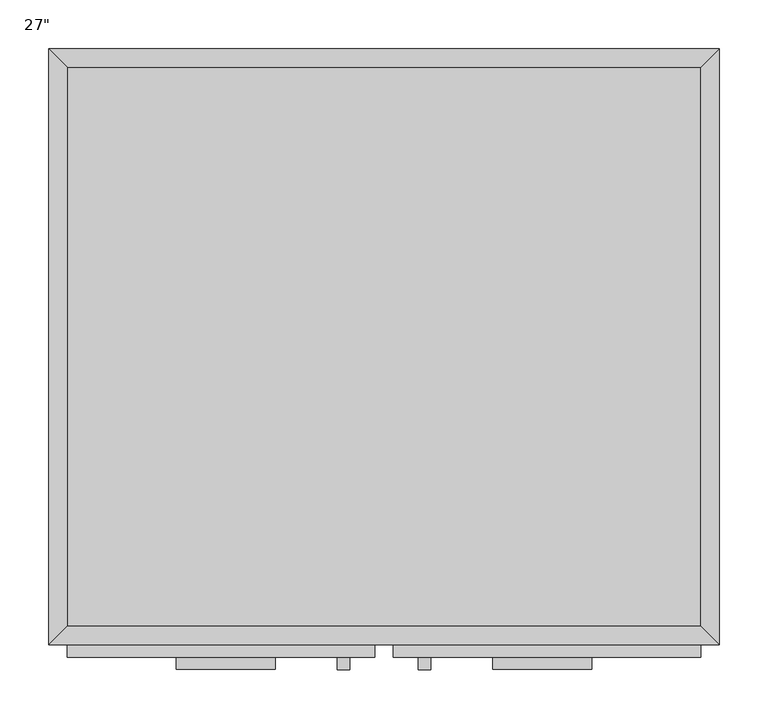
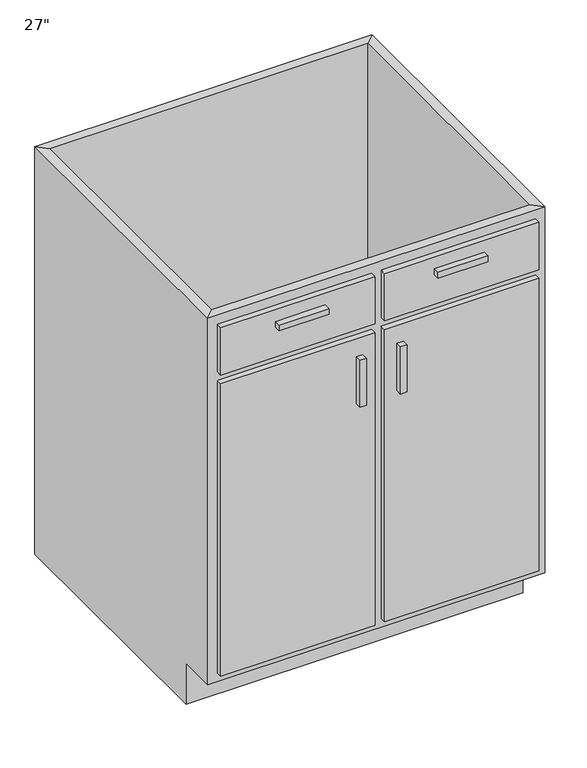
"""IFC4 building model written with IfcOpenShell, lengths in millimetres: furniture geometry."""

from ifc_helpers import new_model, si_unit, frame, origin, place, context, project, spatial, polyline, outline, extrude, faceted_brep, source, transform, mapped, element, save


def furniture_3849fa1a(model_context):
    return source(origin(), model_context, "Body", "SolidModel", [
        faceted_brep([(342.5877049, -590.55, 876.3), (342.5877049, -590.55, 88.9), (-305.1122951, -590.55, 88.9), (-305.1122951, -590.55, 876.3), (-324.1622951, -609.6, 876.3), (361.6377049, -609.6, 876.3), (-324.1622951, -609.6, 88.9), (361.6377049, -609.6, 88.9), (-305.1122951, -533.4, 88.9), (-305.1122951, -19.05, 88.9), (-305.1122951, -19.05, 876.3), (-324.1622951, 0.0, 876.3), (-324.1622951, 0.0, 0.0), (-324.1622951, -533.4, 0.0), (-324.1622951, -533.4, 88.9), (342.5877049, -19.05, 88.9), (342.5877049, -19.05, 876.3), (361.6377049, 0.0, 876.3), (361.6377049, 0.0, 0.0), (342.5877049, -533.4, 88.9), (361.6377049, -533.4, 88.9), (361.6377049, -533.4, 0.0)], [[[0, 1, 2, 3]], [[0, 3, 4, 5]], [[5, 4, 6, 7]], [[2, 1, 7, 6]], [[3, 2, 8, 9, 10]], [[4, 3, 10, 11]], [[6, 4, 11, 12, 13, 14]], [[2, 6, 14, 8]], [[10, 9, 15, 16]], [[11, 10, 16, 17]], [[12, 11, 17, 18]], [[1, 0, 16, 15, 19]], [[0, 5, 17, 16]], [[5, 7, 20, 21, 18, 17]], [[7, 1, 19, 20]], [[8, 19, 15, 9]], [[18, 21, 13, 12]], [[13, 21, 20, 19, 8, 14]]]),
        extrude(outline(polyline([(-92.3872951, -635.0), (-193.9872951, -635.0), (-193.9872951, -622.3), (-92.3872951, -622.3), (-92.3872951, -635.0)])), frame((0.0, 0.0, 819.15), z_axis=(0.0, 0.0, 1.0), x_axis=(1.0, 0.0, 0.0)), (0.0, 0.0, 1.0), 12.7),
        extrude(outline(polyline([(231.4627049, -635.0), (129.8627049, -635.0), (129.8627049, -622.3), (231.4627049, -622.3), (231.4627049, -635.0)])), frame((0.0, 0.0, 819.15), z_axis=(0.0, 0.0, 1.0), x_axis=(1.0, 0.0, 0.0)), (0.0, 0.0, 1.0), 12.7),
        extrude(outline(polyline([(-16.1872951, -635.0), (-28.8872951, -635.0), (-28.8872951, -622.3), (-16.1872951, -622.3), (-16.1872951, -635.0)])), frame((0.0, 0.0, 596.9), z_axis=(0.0, 0.0, 1.0), x_axis=(1.0, 0.0, 0.0)), (0.0, 0.0, 1.0), 101.6),
        extrude(outline(polyline([(66.3627049, -635.0), (53.6627049, -635.0), (53.6627049, -622.3), (66.3627049, -622.3), (66.3627049, -635.0)])), frame((0.0, 0.0, 596.9), z_axis=(0.0, 0.0, 1.0), x_axis=(1.0, 0.0, 0.0)), (0.0, 0.0, 1.0), 101.6),
        extrude(outline(polyline([(342.5877049, -19.05), (342.5877049, -590.55), (-305.1122951, -590.55), (-305.1122951, -19.05), (342.5877049, -19.05)])), frame((0.0, 0.0, 88.9), z_axis=(0.0, 0.0, 1.0), x_axis=(1.0, 0.0, 0.0)), (0.0, 0.0, 1.0), 19.05),
        extrude(outline(polyline([(9.2127049, -622.3), (-305.1122951, -622.3), (-305.1122951, -609.6), (9.2127049, -609.6), (9.2127049, -622.3)])), frame((0.0, 0.0, 755.65), z_axis=(0.0, 0.0, 1.0), x_axis=(1.0, 0.0, 0.0)), (0.0, 0.0, 1.0), 101.6),
        extrude(outline(polyline([(342.5877049, -622.3), (28.2627049, -622.3), (28.2627049, -609.6), (342.5877049, -609.6), (342.5877049, -622.3)])), frame((0.0, 0.0, 755.65), z_axis=(0.0, 0.0, 1.0), x_axis=(1.0, 0.0, 0.0)), (0.0, 0.0, 1.0), 101.6),
        extrude(outline(polyline([(9.2127049, -622.3), (-305.1122951, -622.3), (-305.1122951, -609.6), (9.2127049, -609.6), (9.2127049, -622.3)])), frame((0.0, 0.0, 107.95), z_axis=(0.0, 0.0, 1.0), x_axis=(1.0, 0.0, 0.0)), (0.0, 0.0, 1.0), 628.65),
        extrude(outline(polyline([(342.5877049, -622.3), (28.2627049, -622.3), (28.2627049, -609.6), (342.5877049, -609.6), (342.5877049, -622.3)])), frame((0.0, 0.0, 107.95), z_axis=(0.0, 0.0, 1.0), x_axis=(1.0, 0.0, 0.0)), (0.0, 0.0, 1.0), 628.65),
    ])


if __name__ == "__main__":
    model = new_model("IFC4")
    model_context = context("Model", 3, world=origin())
    ifc_project = project(units=[si_unit("LENGTHUNIT", "METRE", prefix="MILLI")], contexts=[model_context])
    site = spatial("IfcSite", under=ifc_project)
    building = spatial("IfcBuilding", under=site)
    placement = place(None, origin())
    furniture_shape = furniture_3849fa1a(model_context)
    element("IfcFurniture", 1, ObjectType="Base Cabinet-Double Door & 2 Drawer : 27\"", at=placement, inside=building, context=model_context, shape_type="MappedRepresentation", body=[
        mapped(furniture_shape, transform((0.0, 0.0, 0.0), x_axis=(1.0, 0.0, 0.0), y_axis=(0.0, 1.0, 0.0), z_axis=(0.0, 0.0, 1.0))),
    ])
    save(model, "model.ifc")

# Revit data of these elements
# Type "Base Cabinet-Double Door & 2 Drawer : 27\""
#   COBie.Type.CreatedBy = "doug.wood@us.ibm.com"
#   COBie.Type.CreatedOn = "2016-04-14T02:07:23"
#   COBie.Type.Name = "Casework_Base Cabinet-Double Door & 2 Drawer_27\""
#   COBie.Type.Category = "23-40 35 17 47 11 : Kitchen Casework"
#   COBie.Type.Description = "Base Cabinet-Double Door & 2 Drawer_27\""
#   COBie.Type.Manufacturer = ""
#   COBie.Type.ModelNumber = ""
#   Assembly Code = "C1030410"
#   COBie.Type.ReplacementCost = 0
#   Depth = 2' - 0"
#   Height = 2' - 10 1/2"
#   Toe Depth = 0' - 3"
#   Toe Height = 0' - 3 1/2"
#   Width = 2' - 3"
#   COBie.Type = no
#   Cabinet Material = none
#   Door/Drawer Material = none
#   Handle Material = Cabinets - Handles
# Element 1 (IfcFurniture, "Base Cabinet-Double Door & 2 Drawer : 27\"")
#   Materials on its faces: "Cabinets", "Cabinets - Handles"
# Materials
#   "Cabinets - Handles": class "Metal", colour RGB 57 57 57, transparency 0
#   "Cabinets": class "Miscellaneous", colour RGB 249 249 249, transparency 0
